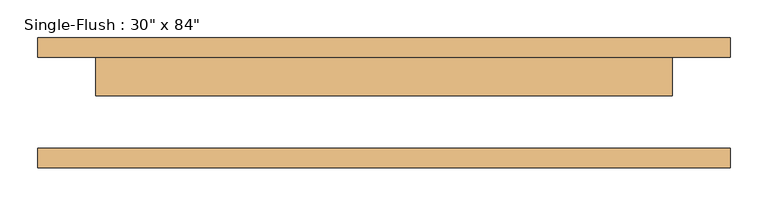
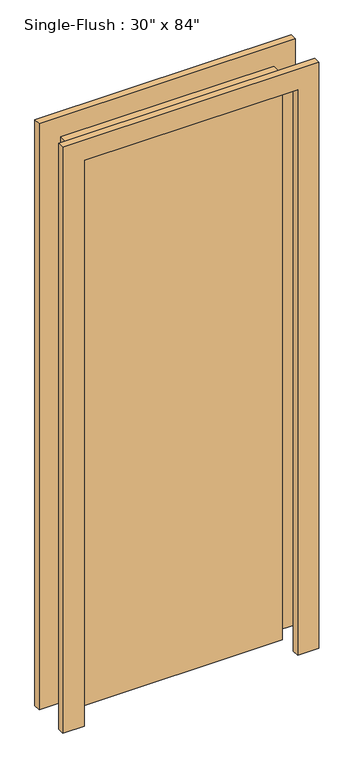
"""IFC4 building model written with IfcOpenShell, lengths in millimetres: door geometry."""

from ifc_helpers import new_model, si_unit, frame, origin, origin_with_axes, place, context, project, spatial, polyline, outline, extrude, source, transform, mapped, element, save


def door_d179b03e(model_context):
    return source(origin(), model_context, "Body", "SweptSolid", [
        extrude(outline(polyline([(2209.8, -457.2), (0.0, -457.2), (0.0, -381.0), (2133.6, -381.0), (2133.6, 381.0), (0.0, 381.0), (0.0, 457.2), (2209.8, 457.2), (2209.8, -457.2)])), frame((0.0, 60.325, 0.0), z_axis=(0.0, 1.0, 0.0), x_axis=(0.0, 0.0, 1.0)), (0.0, 0.0, 1.0), 25.4),
        extrude(outline(polyline([(2209.8, 457.2), (2209.8, -457.2), (0.0, -457.2), (0.0, -381.0), (2133.6, -381.0), (2133.6, 381.0), (0.0, 381.0), (0.0, 457.2), (2209.8, 457.2)])), frame((0.0, -85.725, 0.0), z_axis=(0.0, 1.0, 0.0), x_axis=(0.0, 0.0, 1.0)), (0.0, 0.0, 1.0), 25.4),
        extrude(outline(polyline([(381.0, 9.525), (-381.0, 9.525), (-381.0, 60.325), (381.0, 60.325), (381.0, 9.525)])), origin_with_axes(), (0.0, 0.0, 1.0), 2133.6),
    ])


if __name__ == "__main__":
    model = new_model("IFC4")
    model_context = context("Model", 3, world=origin())
    ifc_project = project(units=[si_unit("LENGTHUNIT", "METRE", prefix="MILLI")], contexts=[model_context])
    site = spatial("IfcSite", under=ifc_project)
    building = spatial("IfcBuilding", under=site)
    placement = place(None, origin())
    door_shape = door_d179b03e(model_context)
    element("IfcDoor", 1, ObjectType="Single-Flush : 30\" x 84\"", at=placement, inside=building, context=model_context, shape_type="MappedRepresentation", body=[
        mapped(door_shape, transform((0.0, 0.0, 0.0), x_axis=(1.0, 0.0, 0.0), y_axis=(0.0, 1.0, 0.0), z_axis=(0.0, 0.0, 1.0))),
    ])
    save(model, "model.ifc")

# Revit data of these elements
# Type "Single-Flush : 30\" x 84\""
#   Type Mark = "4"
#   Construction Type Id = "MDOOR"
#   Assembly Code = "C1020"
#   Analytic Construction = "Metal"
#   Thickness = 0' - 2"
#   Heat Transfer Coefficient (U) = 0.651978 BTU/(h·ft²·°F)
#   Height = 7' - 0"
#   Trim Projection Ext = 0' - 1"
#   Trim Projection Int = 0' - 1"
#   Trim Width = 0' - 3"
#   Width = 2' - 6"
#   Define Thermal Properties by = 1
#   Define Thermal Properties by = 1
#   Door Material = Door - Panel
#   Frame Material = Door - Frame
#   Visual Light Transmittance = 0
#   Solar Heat Gain Coefficient = 0
#   Function = (empty or 0)
#   Wall Closure = (empty or 0)
# Element 1 (IfcDoor, "Single-Flush : 30\" x 84\"")
#   Materials on its faces: "Door - Frame", "Door - Panel"
# Materials
#   "Door - Panel": class "Wood", colour RGB 210 159 95, transparency 0, Cost = 0
#   "Door - Frame": class "Miscellaneous", colour RGB 118 70 51, transparency 0, Cost = 0
